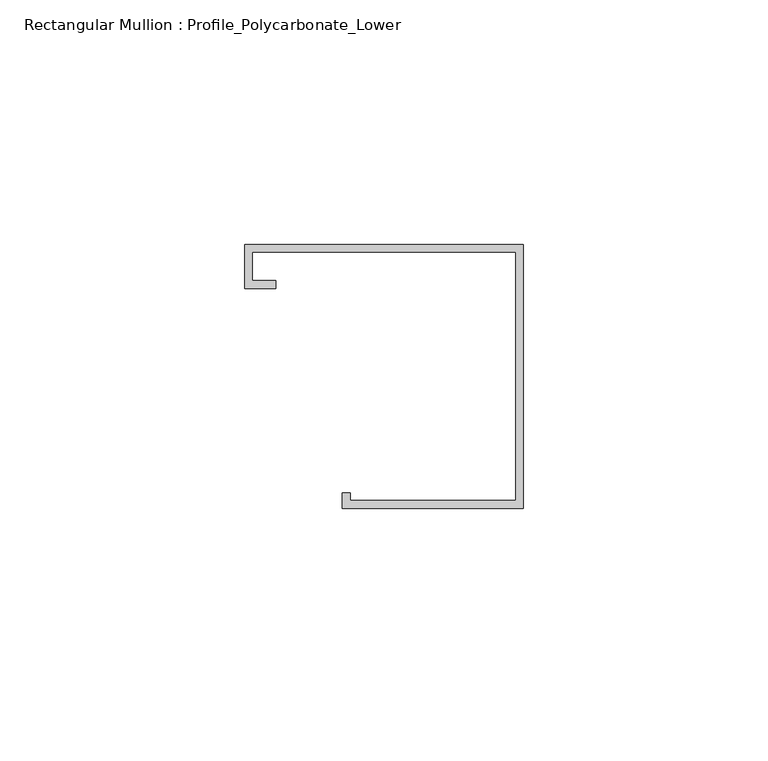
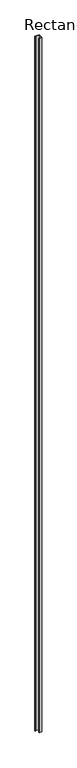
"""IFC4 building model written with IfcOpenShell, lengths in millimetres: member geometry, Rectangular Mullion : Profile_Polycarbonate_Lower."""

import ifcopenshell
import ifcopenshell.guid

model = None  # the IFC model being written
_history = None  # IfcOwnerHistory: only IFC2X3 demands one
_inside = {}  # id of a spatial element -> (the spatial element, [elements in it])
_under = {}  # id of a project, library or spatial element -> (it, [spatial elements below it])
_declared = {}  # id of a project -> (the project, [libraries it declares])
_typed = {}  # id of a type object -> (the type object, [elements of that type])
_made_of = {}  # id of a material, layer set ... -> (it, [elements and type objects made of it])


def new_model(schema):
    """Start an empty IFC model of exactly this schema.

    Asked for "IFC4X3", IfcOpenShell would pick the latest addendum, in which some entities
    have other attributes; the version numbers below select the first issue.
    IFC2X3 requires an IfcOwnerHistory on every rooted entity: one is made here for all.
    """
    global model, _history
    if schema == "IFC4X3":
        model = ifcopenshell.file(schema_version=(4, 3, 0, 0))
    else:
        model = ifcopenshell.file(schema=schema)
    _inside.clear()
    _under.clear()
    _declared.clear()
    _typed.clear()
    _made_of.clear()
    _history = None
    if model.schema == "IFC2X3":
        org = make("IfcOrganization", Name="unknown")
        user = make(
            "IfcPersonAndOrganization",
            ThePerson=make("IfcPerson", FamilyName="unknown"),
            TheOrganization=org,
        )
        app = make(
            "IfcApplication",
            ApplicationDeveloper=org,
            Version="unknown",
            ApplicationFullName="unknown",
            ApplicationIdentifier="unknown",
        )
        _history = make(
            "IfcOwnerHistory",
            OwningUser=user,
            OwningApplication=app,
            ChangeAction="ADDED",
            CreationDate=0,
        )
    return model


def make(cls, **values):
    """One entity of the class cls with the attributes given. An attribute that is None is left unset."""
    return model.create_entity(
        cls, **{name: value for name, value in values.items() if value is not None}
    )


def rooted(cls, **values):
    """An entity with a GlobalId (a new one), such as an element, a storey or a relation."""
    return make(cls, GlobalId=ifcopenshell.guid.new(), OwnerHistory=_history, **values)


def si_unit(unit_type, name, prefix=None):
    """IfcSIUnit, for example si_unit("LENGTHUNIT", "METRE", prefix="MILLI")."""
    return make("IfcSIUnit", UnitType=unit_type, Prefix=prefix, Name=name)


def assignment(units):
    """IfcUnitAssignment: the units of a project."""
    return None if units is None else make("IfcUnitAssignment", Units=units)


def point(xyz):
    """IfcCartesianPoint."""
    return None if xyz is None else make("IfcCartesianPoint", Coordinates=xyz)


def direction(xyz):
    """IfcDirection."""
    return None if xyz is None else make("IfcDirection", DirectionRatios=xyz)


def frame(location, z_axis=None, x_axis=None):
    """IfcAxis2Placement3D, a coordinate frame: its origin and axes. An axis left out is left unset."""
    return make(
        "IfcAxis2Placement3D",
        Location=point(location),
        Axis=direction(z_axis),
        RefDirection=direction(x_axis),
    )


def origin():
    """The frame at (0, 0, 0) with its axes left unset."""
    return frame((0.0, 0.0, 0.0))


def place(relative_to, where):
    """IfcLocalPlacement: puts the frame where relative to a parent placement (None: the world)."""
    return make(
        "IfcLocalPlacement", PlacementRelTo=relative_to, RelativePlacement=where
    )


def context(
    kind, dimensions, precision=None, world=None, true_north=None, identifier=None
):
    """IfcGeometricRepresentationContext, for example the 3D "Model" context."""
    return make(
        "IfcGeometricRepresentationContext",
        ContextIdentifier=identifier,
        ContextType=kind,
        CoordinateSpaceDimension=dimensions,
        Precision=precision,
        WorldCoordinateSystem=world,
        TrueNorth=true_north,
    )


def project(units=None, contexts=None):
    """IfcProject with its units and contexts."""
    return rooted(
        "IfcProject",
        Name="project",
        RepresentationContexts=contexts,
        UnitsInContext=assignment(units),
    )


def spatial(cls, under=None, at=None, **own):
    """A site, building, storey or space (cls), placed at a placement, below another one or the project."""
    s = rooted(cls, ObjectPlacement=at, **own)
    if under is not None:
        _under.setdefault(under.id(), (under, []))[1].append(s)
    return s


def polyline(points):
    """IfcPolyline through the points."""
    return make("IfcPolyline", Points=[point(p) for p in points])


def outline(outer, holes=None, kind="AREA"):
    """IfcArbitraryClosedProfileDef: a profile drawn as a closed curve; with holes, ...WithVoids."""
    if holes is None:
        return make("IfcArbitraryClosedProfileDef", ProfileType=kind, OuterCurve=outer)
    return make(
        "IfcArbitraryProfileDefWithVoids",
        ProfileType=kind,
        OuterCurve=outer,
        InnerCurves=holes,
    )


def extrude(swept, where, along, depth):
    """IfcExtrudedAreaSolid: the profile swept, set in the frame where, extruded along a direction by depth."""
    return make(
        "IfcExtrudedAreaSolid",
        SweptArea=swept,
        Position=where,
        ExtrudedDirection=direction(along),
        Depth=depth,
    )


def shape(context_of_items, identifier, shape_type, items):
    """IfcShapeRepresentation: the items that make up one representation, for example the "Body"."""
    return make(
        "IfcShapeRepresentation",
        ContextOfItems=context_of_items,
        RepresentationIdentifier=identifier,
        RepresentationType=shape_type,
        Items=items,
    )


def source(mapping_origin, context_of_items, identifier, shape_type, items):
    """IfcRepresentationMap: a shape defined once, which mapped items show again and again."""
    return make(
        "IfcRepresentationMap",
        MappingOrigin=mapping_origin,
        MappedRepresentation=shape(context_of_items, identifier, shape_type, items),
    )


def transform(
    local_origin,
    x_axis=None,
    y_axis=None,
    z_axis=None,
    scale=None,
    scale2=None,
    scale3=None,
    uniform=True,
):
    """IfcCartesianTransformationOperator3D, or its non-uniform kind. x_axis, y_axis, z_axis: its Axis1, 2, 3."""
    if uniform:
        return make(
            "IfcCartesianTransformationOperator3D",
            Axis1=direction(x_axis),
            Axis2=direction(y_axis),
            LocalOrigin=point(local_origin),
            Scale=scale,
            Axis3=direction(z_axis),
        )
    return make(
        "IfcCartesianTransformationOperator3DnonUniform",
        Axis1=direction(x_axis),
        Axis2=direction(y_axis),
        LocalOrigin=point(local_origin),
        Scale=scale,
        Axis3=direction(z_axis),
        Scale2=scale2,
        Scale3=scale3,
    )


def mapped(mapping_source, mapping_target):
    """IfcMappedItem: shows the shape of a source again, moved by a transform."""
    return make(
        "IfcMappedItem", MappingSource=mapping_source, MappingTarget=mapping_target
    )


def made_of(thing, what):
    """Note that an element or type object is made of a material, layer set ...; save() writes the relation."""
    if what is not None:
        _made_of.setdefault(what.id(), (what, []))[1].append(thing)
    return thing


def element(
    cls,
    number,
    at=None,
    inside=None,
    cuts=None,
    type_object=None,
    material=None,
    context=None,
    identifier="Body",
    shape_type=None,
    held_by="IfcProductDefinitionShape",
    body=None,
    shapes=None,
    **own,
):
    """One element of the class cls, such as IfcWall. Its Tag is "e" and its number.

    at: its placement. inside: the storey or other place that contains it. cuts: it is an
    opening in that element (IfcRelVoidsElement). A single representation is given by context,
    identifier, shape_type and body (its items); several are given by shapes. held_by: the class
    of the entity that holds the representations. save() writes the other relations.
    """
    e = rooted(cls, Tag="e%d" % number, ObjectPlacement=at, **own)
    if body is not None:
        shapes = [shape(context, identifier, shape_type, body)]
    if shapes is not None:
        e.Representation = make(held_by, Representations=shapes)
    if inside is not None:
        _inside.setdefault(inside.id(), (inside, []))[1].append(e)
    if cuts is not None:
        rooted(
            "IfcRelVoidsElement", RelatingBuildingElement=cuts, RelatedOpeningElement=e
        )
    if type_object is not None:
        _typed.setdefault(type_object.id(), (type_object, []))[1].append(e)
    return made_of(e, material)


def aggregate(whole, parts):
    """IfcRelAggregates: a whole, such as a stair, and the parts it consists of."""
    return rooted("IfcRelAggregates", RelatingObject=whole, RelatedObjects=parts)


def save(model, path):
    """Write the relations noted so far, then the file.

    IfcRelAggregates (storeys below a building ...), IfcRelContainedInSpatialStructure (elements
    in a storey), IfcRelDefinesByType, IfcRelAssociatesMaterial and IfcRelDeclares: one each for
    every whole, place, type object, material and project.
    """
    for whole, parts in _under.values():
        aggregate(whole, parts)
    for where, things in _inside.values():
        rooted(
            "IfcRelContainedInSpatialStructure",
            RelatedElements=things,
            RelatingStructure=where,
        )
    for kind, things in _typed.values():
        rooted("IfcRelDefinesByType", RelatedObjects=things, RelatingType=kind)
    for what, things in _made_of.values():
        rooted("IfcRelAssociatesMaterial", RelatedObjects=things, RelatingMaterial=what)
    for by, libraries in _declared.values():
        rooted("IfcRelDeclares", RelatingContext=by, RelatedDefinitions=libraries)
    model.write(path)


def rectangular_mullion_profile_polycarbonate_lower_4592d3df(model_context):
    return source(origin(), model_context, "Body", "SweptSolid", [
        extrude(outline(polyline([(0.0, 28.984575), (0.0, -25.015825), (-36.9824, -25.015825), (-36.9824, -21.840825), (-35.3949, -21.840825), (-35.3949, -23.428325), (-1.5875, -23.428325), (-1.5875, 27.397075), (-55.4101, 27.397075), (-55.4101, 21.580475), (-50.6476, 21.580475), (-50.6476, 19.992975), (-56.9976, 19.992975), (-56.9976, 28.984575), (0.0, 28.984575)])), frame((0.0, 0.0, -9144.1524), z_axis=(0.0, 0.0, 1.0), x_axis=(1.0, 0.0, 0.0)), (0.0, 0.0, 1.0), 9144.1524),
    ])


if __name__ == "__main__":
    model = new_model("IFC4")
    model_context = context("Model", 3, world=origin())
    ifc_project = project(units=[si_unit("LENGTHUNIT", "METRE", prefix="MILLI")], contexts=[model_context])
    site = spatial("IfcSite", under=ifc_project)
    building = spatial("IfcBuilding", under=site)
    placement = place(None, origin())
    rectangular_mullion_profile_polycarbonate_lower_shape = rectangular_mullion_profile_polycarbonate_lower_4592d3df(model_context)
    element("IfcMember", 1, ObjectType="Rectangular Mullion : Profile_Polycarbonate_Lower", at=placement, inside=building, context=model_context, shape_type="MappedRepresentation", body=[
        mapped(rectangular_mullion_profile_polycarbonate_lower_shape, transform((0.0, 0.0, 0.0), x_axis=(1.0, 0.0, 0.0), y_axis=(0.0, 1.0, 0.0), z_axis=(0.0, 0.0, 1.0))),
    ])
    save(model, "model.ifc")

# Revit data of these elements
# Type "Rectangular Mullion : Profile_Polycarbonate_Lower"
#   built-in parameter 1007322 = 0.177167 (stored number, unit not read)
#   built-in parameter 1007321 = 0 (stored number, unit not read)
#   built-in parameter 1007320 = 0.00520833 (stored number, unit not read)
